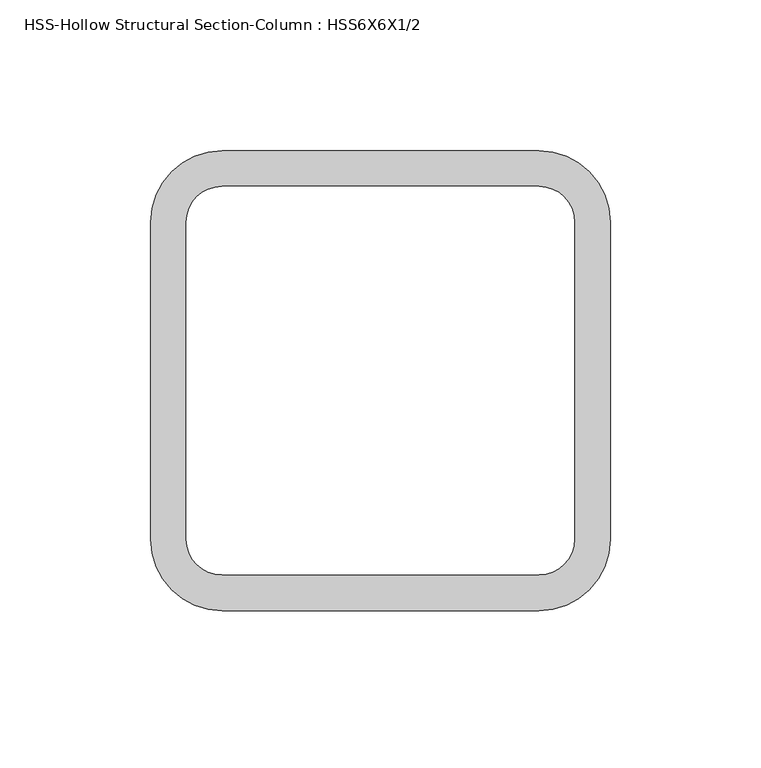
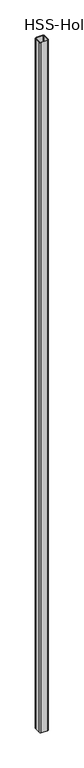
"""IFC4 building model written with IfcOpenShell, lengths in millimetres: column geometry, HSS-Hollow Structural Section-Column : HSS6X6X1/2."""

from ifc_helpers import new_model, si_unit, point, frame_2d, origin, origin_with_axes, place, context, project, spatial, polyline, circle_curve, trimmed, segment, composite_curve, outline, extrude, source, transform, mapped, element, save


def hss_hollow_structural_section_column_hss6x6x1_2_6b59b673(model_context):
    return source(origin(), model_context, "Body", "SweptSolid", [
        extrude(outline(composite_curve([segment(trimmed(circle_curve(frame_2d((52.578, 52.578)), 23.622), [point((52.578, 76.2))], [point((76.2, 52.578))], False, "CARTESIAN"), True, "CONTINUOUS"), segment(polyline([(76.2, 52.578), (76.2, -52.578)]), True, "CONTINUOUS"), segment(trimmed(circle_curve(frame_2d((52.578, -52.578)), 23.622), [point((76.2, -52.578))], [point((52.578, -76.2))], False, "CARTESIAN"), True, "CONTINUOUS"), segment(polyline([(52.578, -76.2), (-52.578, -76.2)]), True, "CONTINUOUS"), segment(trimmed(circle_curve(frame_2d((-52.578, -52.578)), 23.622), [point((-52.578, -76.2))], [point((-76.2, -52.578))], False, "CARTESIAN"), True, "CONTINUOUS"), segment(polyline([(-76.2, -52.578), (-76.2, 52.578)]), True, "CONTINUOUS"), segment(trimmed(circle_curve(frame_2d((-52.578, 52.578)), 23.622), [point((-76.2, 52.578))], [point((-52.578, 76.2))], False, "CARTESIAN"), True, "CONTINUOUS"), segment(polyline([(-52.578, 76.2), (52.578, 76.2)]), True, "CONTINUOUS")], self_intersect=False), holes=[composite_curve([segment(polyline([(52.578, 64.389), (-52.578, 64.389)]), True, "CONTINUOUS"), segment(trimmed(circle_curve(frame_2d((-52.578, 52.578)), 11.811), [point((-52.578, 64.389))], [point((-64.389, 52.578))], True, "CARTESIAN"), True, "CONTINUOUS"), segment(polyline([(-64.389, 52.578), (-64.389, -52.578)]), True, "CONTINUOUS"), segment(trimmed(circle_curve(frame_2d((-52.578, -52.578)), 11.811), [point((-64.389, -52.578))], [point((-52.578, -64.389))], True, "CARTESIAN"), True, "CONTINUOUS"), segment(polyline([(-52.578, -64.389), (52.578, -64.389)]), True, "CONTINUOUS"), segment(trimmed(circle_curve(frame_2d((52.578, -52.578)), 11.811), [point((52.578, -64.389))], [point((64.389, -52.578))], True, "CARTESIAN"), True, "CONTINUOUS"), segment(polyline([(64.389, -52.578), (64.389, 52.578)]), True, "CONTINUOUS"), segment(trimmed(circle_curve(frame_2d((52.578, 52.578)), 11.811), [point((64.389, 52.578))], [point((52.578, 64.389))], True, "CARTESIAN"), True, "CONTINUOUS")], self_intersect=False)]), origin_with_axes(), (0.0, 0.0, 1.0), 12547.6),
    ])


if __name__ == "__main__":
    model = new_model("IFC4")
    model_context = context("Model", 3, world=origin())
    ifc_project = project(units=[si_unit("LENGTHUNIT", "METRE", prefix="MILLI")], contexts=[model_context])
    site = spatial("IfcSite", under=ifc_project)
    building = spatial("IfcBuilding", under=site)
    placement = place(None, origin())
    hss_hollow_structural_section_column_hss6x6x1_2_shape = hss_hollow_structural_section_column_hss6x6x1_2_6b59b673(model_context)
    element("IfcColumn", 1, ObjectType="HSS-Hollow Structural Section-Column : HSS6X6X1/2", at=placement, inside=building, context=model_context, shape_type="MappedRepresentation", body=[
        mapped(hss_hollow_structural_section_column_hss6x6x1_2_shape, transform((0.0, 0.0, 0.0), x_axis=(1.0, 0.0, 0.0), y_axis=(0.0, 1.0, 0.0), z_axis=(0.0, 0.0, 1.0))),
    ])
    save(model, "model.ifc")

# Revit data of these elements
# Type "HSS-Hollow Structural Section-Column : HSS6X6X1/2"
#   Assembly Code = "B10"
#   Shape = "Square"
#   W = 35.1
#   Ht = 0' - 6"
#   b = 0' - 6"
#   kr = 0' - 0.93"
#   t = 0' - 0.465"
#   A = 0.0676389 SF
#   Structural Material [instance default] = Steel ASTM A500, Grade B, Rectangular and Square
# Element 1 (IfcColumn, "HSS-Hollow Structural Section-Column : HSS6X6X1/2")
#   Materials on its faces: "Steel ASTM A500, Grade B, Rectangular and Square"
# Materials
#   "Steel ASTM A500, Grade B, Rectangular and Square": class "Metal", colour RGB 199 199 199, transparency 0, Description = "Carbon steel", Cost = 0
